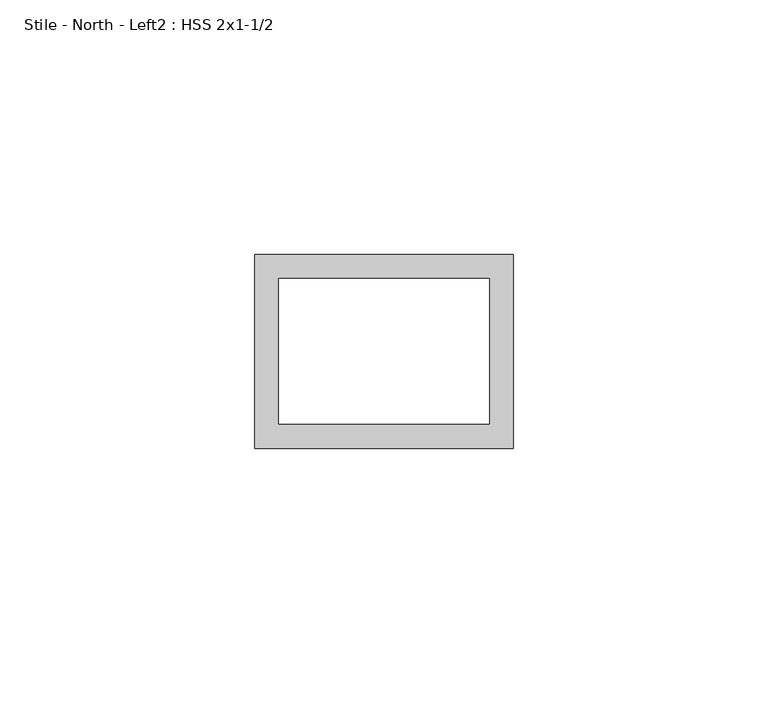
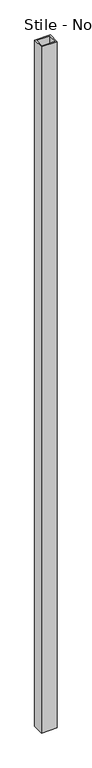
"""IFC4 building model written with IfcOpenShell, lengths in millimetres: proxy geometry, Stile - North - Left2 : HSS 2x1-1/2."""

from ifc_helpers import new_model, si_unit, frame, origin, place, context, project, spatial, polyline, outline, extrude, source, transform, mapped, element, save


def stile_north_left2_hss_2x1_1_2_25622c15(model_context):
    return source(origin(), model_context, "Body", "SweptSolid", [
        extrude(outline(polyline([(587365.8934739, -531785.2663841), (587416.6934739, -531785.2663841), (587416.6934739, -531823.3663841), (587365.8934739, -531823.3663841), (587365.8934739, -531785.2663841)]), holes=[polyline([(587370.6559739, -531790.0288841), (587370.6559739, -531818.6038841), (587411.9309739, -531818.6038841), (587411.9309739, -531790.0288841), (587370.6559739, -531790.0288841)])]), frame((0.0, 0.0, 50.8), z_axis=(0.0, 0.0, 1.0), x_axis=(1.0, 0.0, 0.0)), (0.0, 0.0, 1.0), 2349.5),
    ])


if __name__ == "__main__":
    model = new_model("IFC4")
    model_context = context("Model", 3, world=origin())
    ifc_project = project(units=[si_unit("LENGTHUNIT", "METRE", prefix="MILLI")], contexts=[model_context])
    site = spatial("IfcSite", under=ifc_project)
    building = spatial("IfcBuilding", under=site)
    placement = place(None, origin())
    stile_north_left2_hss_2x1_1_2_shape = stile_north_left2_hss_2x1_1_2_25622c15(model_context)
    element("IfcBuildingElementProxy", 1, Name="Stile - North - Left2 : HSS 2x1-1/2", ObjectType="Stile - North - Left2 : HSS 2x1-1/2", at=placement, inside=building, context=model_context, shape_type="MappedRepresentation", body=[
        mapped(stile_north_left2_hss_2x1_1_2_shape, transform((0.0, 0.0, 0.0), x_axis=(1.0, 0.0, 0.0), y_axis=(0.0, 1.0, 0.0), z_axis=(0.0, 0.0, 1.0))),
    ])
    save(model, "model.ifc")

# Revit data of these elements
# Element 1 (IfcBuildingElementProxy, "Stile - North - Left2 : HSS 2x1-1/2")
#   Materials on its faces: "1-1/2\"X2\" GALV. STL HSS TUBING"
# Materials
#   "1-1/2\"X2\" GALV. STL HSS TUBING": class "Generic", colour RGB 211 211 207, transparency 0, Cost = 0
